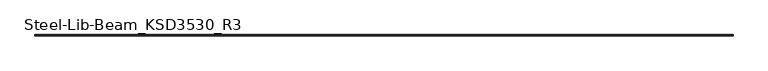
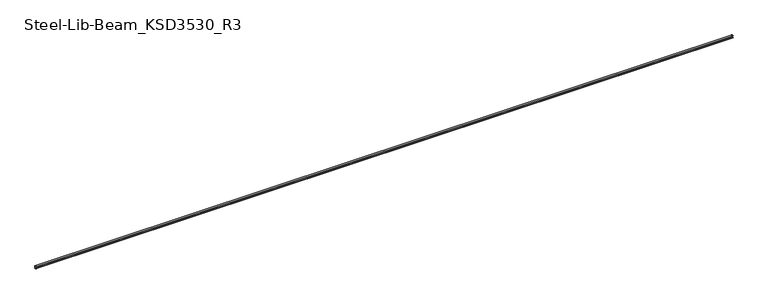
"""IFC4 building model written with IfcOpenShell, lengths in millimetres: beam geometry, Steel-Lib-Beam_KSD3530_R3 : BMS291_C-150×75x20x4.5."""

from ifc_helpers import new_model, si_unit, point, frame, frame_2d, origin, place, context, project, spatial, polyline, circle_curve, trimmed, segment, composite_curve, outline, extrude, source, transform, mapped, element, save


def steel_lib_beam_ksd3530_r3_6bb2b8aa(model_context):
    return source(origin(), model_context, "Body", "SweptSolid", [
        extrude(outline(composite_curve([segment(trimmed(circle_curve(frame_2d((-41.0, 66.0)), 9.0), [point((-50.0, 66.0))], [point((-41.0, 75.0))], False, "CARTESIAN"), True, "CONTINUOUS"), segment(polyline([(-41.0, 75.0), (16.0, 75.0)]), True, "CONTINUOUS"), segment(trimmed(circle_curve(frame_2d((16.0, 66.0)), 9.0), [point((16.0, 75.0))], [point((25.0, 66.0))], False, "CARTESIAN"), True, "CONTINUOUS"), segment(polyline([(25.0, 66.0), (25.0, -66.0)]), True, "CONTINUOUS"), segment(trimmed(circle_curve(frame_2d((16.0, -66.0)), 9.0), [point((25.0, -66.0))], [point((16.0, -75.0))], False, "CARTESIAN"), True, "CONTINUOUS"), segment(polyline([(16.0, -75.0), (-41.0, -75.0)]), True, "CONTINUOUS"), segment(trimmed(circle_curve(frame_2d((-41.0, -66.0)), 9.0), [point((-41.0, -75.0))], [point((-50.0, -66.0))], False, "CARTESIAN"), True, "CONTINUOUS"), segment(polyline([(-50.0, -66.0), (-50.0, -55.0), (-45.5, -55.0), (-45.5, -66.0)]), True, "CONTINUOUS"), segment(trimmed(circle_curve(frame_2d((-41.0, -66.0)), 4.5), [point((-45.5, -66.0))], [point((-41.0, -70.5))], True, "CARTESIAN"), True, "CONTINUOUS"), segment(polyline([(-41.0, -70.5), (16.0, -70.5)]), True, "CONTINUOUS"), segment(trimmed(circle_curve(frame_2d((16.0, -66.0)), 4.5), [point((16.0, -70.5))], [point((20.5, -66.0))], True, "CARTESIAN"), True, "CONTINUOUS"), segment(polyline([(20.5, -66.0), (20.5, 66.0)]), True, "CONTINUOUS"), segment(trimmed(circle_curve(frame_2d((16.0, 66.0)), 4.5), [point((20.5, 66.0))], [point((16.0, 70.5))], True, "CARTESIAN"), True, "CONTINUOUS"), segment(polyline([(16.0, 70.5), (-41.0, 70.5)]), True, "CONTINUOUS"), segment(trimmed(circle_curve(frame_2d((-41.0, 66.0)), 4.5), [point((-41.0, 70.5))], [point((-45.5, 66.0))], True, "CARTESIAN"), True, "CONTINUOUS"), segment(polyline([(-45.5, 66.0), (-45.5, 55.0), (-50.0, 55.0), (-50.0, 66.0)]), True, "CONTINUOUS")], self_intersect=False)), frame((-20557.5, 0.0, 0.0), z_axis=(1.0, 0.0, 0.0), x_axis=(0.0, 1.0, 0.0)), (0.0, 0.0, 1.0), 41115.0),
    ])


if __name__ == "__main__":
    model = new_model("IFC4")
    model_context = context("Model", 3, world=origin())
    ifc_project = project(units=[si_unit("LENGTHUNIT", "METRE", prefix="MILLI")], contexts=[model_context])
    site = spatial("IfcSite", under=ifc_project)
    building = spatial("IfcBuilding", under=site)
    placement = place(None, origin())
    steel_lib_beam_ksd3530_r3_shape = steel_lib_beam_ksd3530_r3_6bb2b8aa(model_context)
    element("IfcBeam", 1, ObjectType="Steel-Lib-Beam_KSD3530_R3 : BMS291_C-150×75x20x4.5", at=placement, inside=building, context=model_context, shape_type="MappedRepresentation", body=[
        mapped(steel_lib_beam_ksd3530_r3_shape, transform((0.0, 0.0, 0.0), x_axis=(1.0, 0.0, 0.0), y_axis=(0.0, 1.0, 0.0), z_axis=(0.0, 0.0, 1.0))),
    ])
    save(model, "model.ifc")

# Revit data of these elements
# Type "Steel-Lib-Beam_KSD3530_R3 : BMS291_C-150×75x20x4.5"
#   Keynote = "C-150×75x20x4.5"
#   SteelWeight = "Light"
#   x = 0.0250 m
#   t1 = 0.0090 m
#   t = 0.0045 m
#   Surface Area = 0.629834 m²/m
#   Section Area = 13.9688 cm²
#   Mass per Unit Length = 10.9655 kg/m
#   C = 0.0200 m
#   A = 0.0750 m
#   Length [instance default] = 1.5000 m
#   H = 0.1500 m
#   hec_material4 [instance default] = none
#   hec_material3 [instance default] = none
#   hec_material2 [instance default] = none
#   hec_material1 [instance default] = none
#   Structural Material [instance default] = Metal - Steel - Light Gauge
#   Assembly Code = ""
# Element 1 (IfcBeam, "Steel-Lib-Beam_KSD3530_R3 : BMS291_C-150×75x20x4.5")
#   Structural Material = none
# Materials
#   "Metal - Steel - Light Gauge": class "Metal", colour RGB 247 247 247, transparency 0
